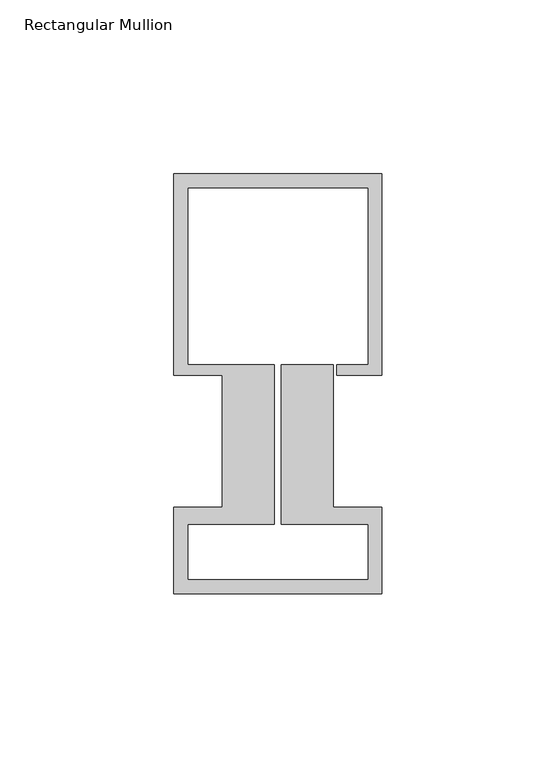
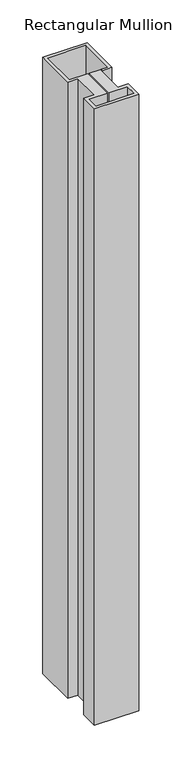
"""IFC4 building model written with IfcOpenShell, lengths in millimetres: member geometry, Rectangular Mullion : Schueco_FWS-60-SI_Tran_CovCap-20mm_Tran-55mm."""

from ifc_helpers import new_model, si_unit, frame, origin, place, context, project, spatial, polyline, outline, extrude, source, transform, mapped, element, save


def rectangular_mullion_9ae110a3(model_context):
    return source(origin(), model_context, "Body", "SweptSolid", [
        extrude(outline(polyline([(-60.0, 96.0), (0.0, 96.0), (0.0, 38.0), (-13.0, 38.0), (-13.0, 41.0), (-4.0, 41.0), (-4.0, 92.0), (-56.0, 92.0), (-56.0, 41.0), (-31.0, 41.0), (-31.0, -5.0), (-56.0, -5.0), (-56.0, -21.0), (-4.0, -21.0), (-4.0, -5.0), (-29.0, -5.0), (-29.0, 41.0), (-14.0, 41.0), (-14.0, -0.1), (0.0, -0.1), (0.0, -25.0), (-60.0, -25.0), (-60.0, -0.1), (-46.0, -0.1), (-46.0, 38.0), (-60.0, 38.0), (-60.0, 96.0)])), frame((0.0, 0.0, -880.0), z_axis=(0.0, 0.0, 1.0), x_axis=(1.0, 0.0, 0.0)), (0.0, 0.0, 1.0), 880.0),
    ])


if __name__ == "__main__":
    model = new_model("IFC4")
    model_context = context("Model", 3, world=origin())
    ifc_project = project(units=[si_unit("LENGTHUNIT", "METRE", prefix="MILLI")], contexts=[model_context])
    site = spatial("IfcSite", under=ifc_project)
    building = spatial("IfcBuilding", under=site)
    placement = place(None, origin())
    rectangular_mullion_shape = rectangular_mullion_9ae110a3(model_context)
    element("IfcMember", 1, ObjectType="Rectangular Mullion : Schueco_FWS-60-SI_Tran_CovCap-20mm_Tran-55mm", at=placement, inside=building, context=model_context, shape_type="MappedRepresentation", body=[
        mapped(rectangular_mullion_shape, transform((0.0, 0.0, 0.0), x_axis=(1.0, 0.0, 0.0), y_axis=(0.0, 1.0, 0.0), z_axis=(0.0, 0.0, 1.0))),
    ])
    save(model, "model.ifc")

# Revit data of these elements
# Type "Rectangular Mullion : Schueco_FWS-60-SI_Tran_CovCap-20mm_Tran-55mm"
#   Model = "FWS 60.SI"
#   Manufacturer = "Schueco International KG"
#   Type Comments = "Transom"
#   Schueco thermal insulation standard = "Suitable for passive houses"
#   Burglar resistance = "RC 3"
#   Thermal insulation = "to 0.70 W/(m²K)"
#   built-in parameter 1007322 = 0.396982 (stored number, unit not read)
#   built-in parameter 1007321 = 0.0524934 (stored number, unit not read)
#   built-in parameter 1007320 = 0.0524934 (stored number, unit not read)
# Element 1 (IfcMember, "Rectangular Mullion : Schueco_FWS-60-SI_Tran_CovCap-20mm_Tran-55mm")
#   Materials on its faces: "Alu"
# Materials
#   "Alu": class "Glas", colour RGB 140 140 140, transparency 0
